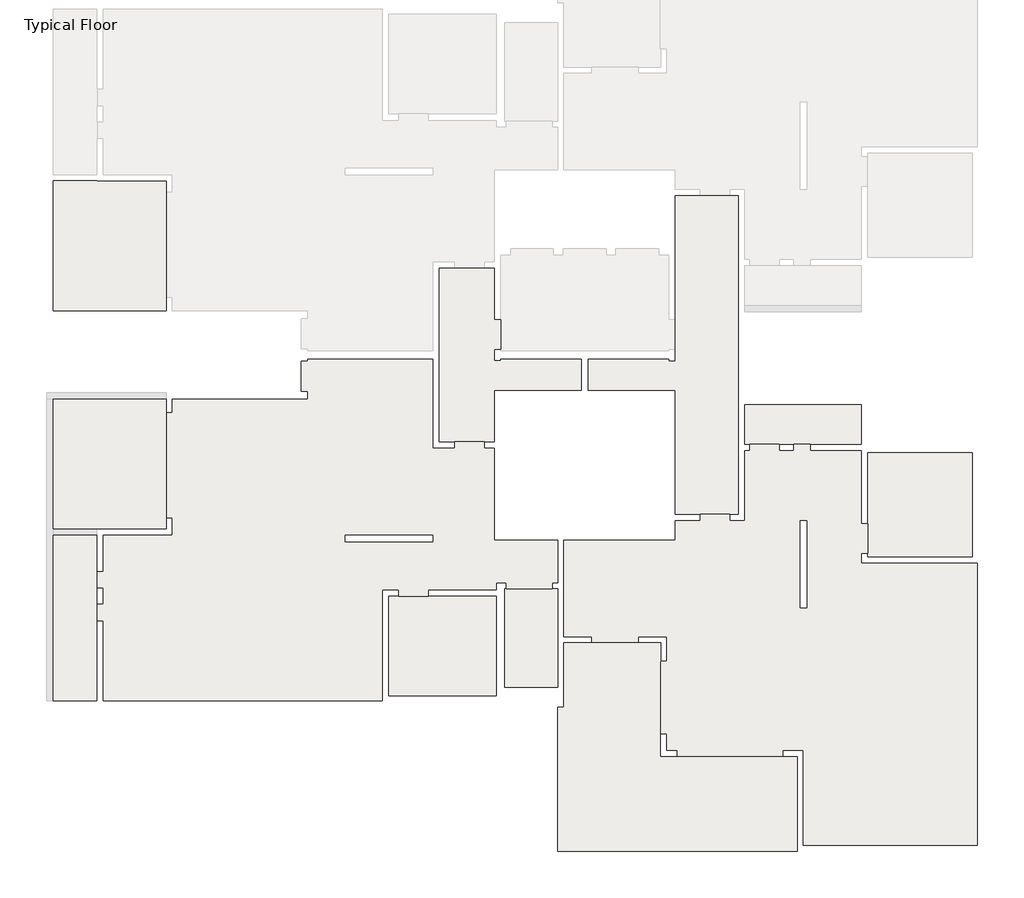
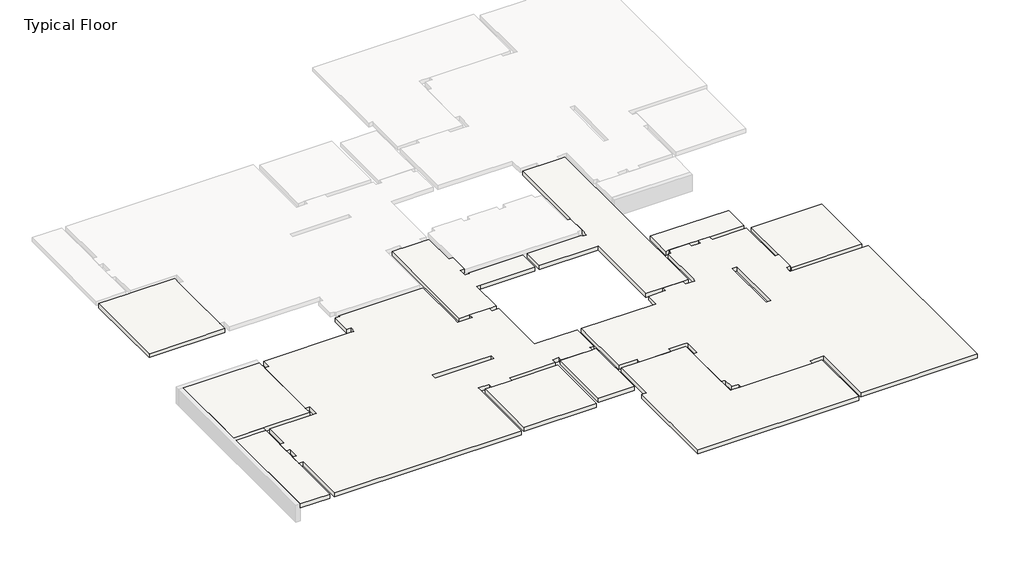
# One storey, part 1 of 2: 12 slabs.
"""IFC4 building model written with IfcOpenShell, lengths in millimetres."""

import ifcopenshell
import ifcopenshell.guid

model = None  # the IFC model being written
_history = None  # IfcOwnerHistory: only IFC2X3 demands one
_inside = {}  # id of a spatial element -> (the spatial element, [elements in it])
_under = {}  # id of a project, library or spatial element -> (it, [spatial elements below it])
_declared = {}  # id of a project -> (the project, [libraries it declares])
_typed = {}  # id of a type object -> (the type object, [elements of that type])
_made_of = {}  # id of a material, layer set ... -> (it, [elements and type objects made of it])


def new_model(schema):
    """Start an empty IFC model of exactly this schema.

    Asked for "IFC4X3", IfcOpenShell would pick the latest addendum, in which some entities
    have other attributes; the version numbers below select the first issue.
    IFC2X3 requires an IfcOwnerHistory on every rooted entity: one is made here for all.
    """
    global model, _history
    if schema == "IFC4X3":
        model = ifcopenshell.file(schema_version=(4, 3, 0, 0))
    else:
        model = ifcopenshell.file(schema=schema)
    _inside.clear()
    _under.clear()
    _declared.clear()
    _typed.clear()
    _made_of.clear()
    _history = None
    if model.schema == "IFC2X3":
        org = make("IfcOrganization", Name="unknown")
        user = make(
            "IfcPersonAndOrganization",
            ThePerson=make("IfcPerson", FamilyName="unknown"),
            TheOrganization=org,
        )
        app = make(
            "IfcApplication",
            ApplicationDeveloper=org,
            Version="unknown",
            ApplicationFullName="unknown",
            ApplicationIdentifier="unknown",
        )
        _history = make(
            "IfcOwnerHistory",
            OwningUser=user,
            OwningApplication=app,
            ChangeAction="ADDED",
            CreationDate=0,
        )
    return model


def make(cls, **values):
    """One entity of the class cls with the attributes given. An attribute that is None is left unset."""
    return model.create_entity(
        cls, **{name: value for name, value in values.items() if value is not None}
    )


def rooted(cls, **values):
    """An entity with a GlobalId (a new one), such as an element, a storey or a relation."""
    return make(cls, GlobalId=ifcopenshell.guid.new(), OwnerHistory=_history, **values)


def si_unit(unit_type, name, prefix=None):
    """IfcSIUnit, for example si_unit("LENGTHUNIT", "METRE", prefix="MILLI")."""
    return make("IfcSIUnit", UnitType=unit_type, Prefix=prefix, Name=name)


def assignment(units):
    """IfcUnitAssignment: the units of a project."""
    return None if units is None else make("IfcUnitAssignment", Units=units)


def point(xyz):
    """IfcCartesianPoint."""
    return None if xyz is None else make("IfcCartesianPoint", Coordinates=xyz)


def direction(xyz):
    """IfcDirection."""
    return None if xyz is None else make("IfcDirection", DirectionRatios=xyz)


def frame(location, z_axis=None, x_axis=None):
    """IfcAxis2Placement3D, a coordinate frame: its origin and axes. An axis left out is left unset."""
    return make(
        "IfcAxis2Placement3D",
        Location=point(location),
        Axis=direction(z_axis),
        RefDirection=direction(x_axis),
    )


def origin():
    """The frame at (0, 0, 0) with its axes left unset."""
    return frame((0.0, 0.0, 0.0))


def place(relative_to, where):
    """IfcLocalPlacement: puts the frame where relative to a parent placement (None: the world)."""
    return make(
        "IfcLocalPlacement", PlacementRelTo=relative_to, RelativePlacement=where
    )


def context(
    kind, dimensions, precision=None, world=None, true_north=None, identifier=None
):
    """IfcGeometricRepresentationContext, for example the 3D "Model" context."""
    return make(
        "IfcGeometricRepresentationContext",
        ContextIdentifier=identifier,
        ContextType=kind,
        CoordinateSpaceDimension=dimensions,
        Precision=precision,
        WorldCoordinateSystem=world,
        TrueNorth=true_north,
    )


def project(units=None, contexts=None):
    """IfcProject with its units and contexts."""
    return rooted(
        "IfcProject",
        Name="project",
        RepresentationContexts=contexts,
        UnitsInContext=assignment(units),
    )


def spatial(cls, under=None, at=None, **own):
    """A site, building, storey or space (cls), placed at a placement, below another one or the project."""
    s = rooted(cls, ObjectPlacement=at, **own)
    if under is not None:
        _under.setdefault(under.id(), (under, []))[1].append(s)
    return s


def faces_of(points, faces, orient=None, outer=None):
    """IfcFace entities. A face is a list of loops; a loop is a list of indices into points, from 0.

    orient and outer hold one flag for each loop. By default every Orientation is true, the
    first loop of a face is its IfcFaceOuterBound and the others are IfcFaceBound.
    """
    made = []
    for i, loops in enumerate(faces):
        bounds = []
        for j, loop in enumerate(loops):
            is_outer = j == 0 if outer is None else outer[i][j]
            bounds.append(
                make(
                    "IfcFaceOuterBound" if is_outer else "IfcFaceBound",
                    Bound=make("IfcPolyLoop", Polygon=[points[k] for k in loop]),
                    Orientation=True if orient is None else orient[i][j],
                )
            )
        made.append(make("IfcFace", Bounds=bounds))
    return made


def faceted_brep(points, faces, orient=None, outer=None, voids=None):
    """IfcFacetedBrep: a solid bounded by flat faces; with voids (closed shells), ...WithVoids."""
    shared = [point(p) for p in points]
    hull = make("IfcClosedShell", CfsFaces=faces_of(shared, faces, orient, outer))
    if voids is None:
        return make("IfcFacetedBrep", Outer=hull)
    return make(
        "IfcFacetedBrepWithVoids",
        Outer=hull,
        Voids=[
            make(cls, CfsFaces=faces_of(shared, fs, o, b)) for cls, fs, o, b in voids
        ],
    )


def shape(context_of_items, identifier, shape_type, items):
    """IfcShapeRepresentation: the items that make up one representation, for example the "Body"."""
    return make(
        "IfcShapeRepresentation",
        ContextOfItems=context_of_items,
        RepresentationIdentifier=identifier,
        RepresentationType=shape_type,
        Items=items,
    )


def made_of(thing, what):
    """Note that an element or type object is made of a material, layer set ...; save() writes the relation."""
    if what is not None:
        _made_of.setdefault(what.id(), (what, []))[1].append(thing)
    return thing


def element(
    cls,
    number,
    at=None,
    inside=None,
    cuts=None,
    type_object=None,
    material=None,
    context=None,
    identifier="Body",
    shape_type=None,
    held_by="IfcProductDefinitionShape",
    body=None,
    shapes=None,
    **own,
):
    """One element of the class cls, such as IfcWall. Its Tag is "e" and its number.

    at: its placement. inside: the storey or other place that contains it. cuts: it is an
    opening in that element (IfcRelVoidsElement). A single representation is given by context,
    identifier, shape_type and body (its items); several are given by shapes. held_by: the class
    of the entity that holds the representations. save() writes the other relations.
    """
    e = rooted(cls, Tag="e%d" % number, ObjectPlacement=at, **own)
    if body is not None:
        shapes = [shape(context, identifier, shape_type, body)]
    if shapes is not None:
        e.Representation = make(held_by, Representations=shapes)
    if inside is not None:
        _inside.setdefault(inside.id(), (inside, []))[1].append(e)
    if cuts is not None:
        rooted(
            "IfcRelVoidsElement", RelatingBuildingElement=cuts, RelatedOpeningElement=e
        )
    if type_object is not None:
        _typed.setdefault(type_object.id(), (type_object, []))[1].append(e)
    return made_of(e, material)


def aggregate(whole, parts):
    """IfcRelAggregates: a whole, such as a stair, and the parts it consists of."""
    return rooted("IfcRelAggregates", RelatingObject=whole, RelatedObjects=parts)


def save(model, path):
    """Write the relations noted so far, then the file.

    IfcRelAggregates (storeys below a building ...), IfcRelContainedInSpatialStructure (elements
    in a storey), IfcRelDefinesByType, IfcRelAssociatesMaterial and IfcRelDeclares: one each for
    every whole, place, type object, material and project.
    """
    for whole, parts in _under.values():
        aggregate(whole, parts)
    for where, things in _inside.values():
        rooted(
            "IfcRelContainedInSpatialStructure",
            RelatedElements=things,
            RelatingStructure=where,
        )
    for kind, things in _typed.values():
        rooted("IfcRelDefinesByType", RelatedObjects=things, RelatingType=kind)
    for what, things in _made_of.values():
        rooted("IfcRelAssociatesMaterial", RelatedObjects=things, RelatingMaterial=what)
    for by, libraries in _declared.values():
        rooted("IfcRelDeclares", RelatingContext=by, RelatedDefinitions=libraries)
    model.write(path)


model = new_model("IFC4")

# Units and contexts
model_context = context("Model", 3, world=origin())
ifc_project = project(units=[si_unit("LENGTHUNIT", "METRE", prefix="MILLI")], contexts=[model_context])

# Site, building, storey
site = spatial("IfcSite", under=ifc_project)
building = spatial("IfcBuilding", under=site)
storey = spatial("IfcBuildingStorey", under=building, Name="Typical Floor", Elevation=3000.0)

# Slabs
placement = place(None, origin())
element("IfcSlab", 1, ObjectType="19", at=placement, inside=storey, context=model_context, shape_type="Brep", body=[
    faceted_brep([(7776.7577342, 16126.4707233, 2810.0), (4344.3623691, 16126.4707233, 2810.0), (4344.3623691, 20058.0459905, 2810.0), (4344.3623691, 20073.0459905, 2810.0), (5676.0285364, 20073.0459905, 2810.0), (5676.0285364, 20058.0459905, 2810.0), (7776.7577342, 20058.0459905, 2810.0), (7776.7577342, 19727.6893828, 2810.0), (7776.7577342, 16527.889163, 2810.0), (4344.3623691, 16126.4707233, 3000.0), (7776.7577342, 16126.4707233, 3000.0), (7776.7577342, 16527.889163, 3000.0), (7776.7577342, 19727.6893828, 3000.0), (7776.7577342, 20058.0459905, 3000.0), (5866.0285364, 20058.0459905, 3000.0), (5676.0285364, 20058.0459905, 3000.0), (5676.0285364, 20073.0459905, 3000.0), (4344.3623691, 20073.0459905, 3000.0)], [[[0, 1, 2, 3, 4, 5, 6, 7, 8]], [[9, 10, 11, 12, 13, 14, 15, 16, 17]], [[3, 17, 16, 4]], [[10, 0, 8, 7, 6, 13, 12, 11]], [[1, 0, 10, 9]], [[3, 2, 1, 9, 17]], [[5, 15, 14, 13, 6]], [[15, 5, 4, 16]]]),
])
element("IfcSlab", 2, ObjectType="19", at=placement, inside=storey, context=model_context, shape_type="Brep", body=[
    faceted_brep([(4344.3623691, 9503.461034, 2810.0), (4344.3623691, 13435.0363012, 2810.0), (7776.7577342, 13435.0363012, 2810.0), (7776.7577342, 13033.6178615, 2810.0), (7776.7577342, 9833.8176417, 2810.0), (7776.7577342, 9503.461034, 2810.0), (4344.3623691, 9503.461034, 3000.0), (5676.0285364, 9503.461034, 3000.0), (5866.0285364, 9503.461034, 3000.0), (7776.7577342, 9503.461034, 3000.0), (7776.7577342, 9833.8176417, 3000.0), (7776.7577342, 13033.6178615, 3000.0), (7776.7577342, 13435.0363012, 3000.0), (4344.3623691, 13435.0363012, 3000.0)], [[[0, 1, 2, 3, 4, 5]], [[6, 7, 8, 9, 10, 11, 12, 13]], [[0, 5, 9, 8, 7, 6]], [[5, 4, 3, 2, 12, 11, 10, 9]], [[2, 1, 13, 12]], [[1, 0, 6, 13]]]),
])
element("IfcSlab", 3, ObjectType="19", at=placement, inside=storey, context=model_context, shape_type="Brep", body=[
    faceted_brep([(5676.0285364, 4280.8870961, 2810.0), (4344.3623691, 4280.8870961, 2810.0), (4344.3623691, 9303.461034, 2810.0), (4344.3623691, 9308.461034, 2810.0), (5676.0285364, 9308.461034, 2810.0), (5676.0285364, 9303.461034, 2810.0), (5676.0285364, 8207.3295478, 2810.0), (5676.0285364, 7708.0987786, 2810.0), (5676.0285364, 7208.8680094, 2810.0), (5676.0285364, 6709.6372401, 2810.0), (5676.0285364, 4280.8870961, 3000.0), (5676.0285364, 6709.6372401, 3000.0), (5676.0285364, 7208.8680094, 3000.0), (5676.0285364, 7708.0987786, 3000.0), (5676.0285364, 8207.3295478, 3000.0), (5676.0285364, 9308.461034, 3000.0), (4344.3623691, 9308.461034, 3000.0), (4344.3623691, 4280.8870961, 3000.0)], [[[0, 1, 2, 3, 4, 5, 6, 7, 8, 9]], [[10, 11, 12, 13, 14, 15, 16, 17]], [[0, 9, 8, 7, 6, 5, 4, 15, 14, 13, 12, 11, 10]], [[4, 3, 16, 15]], [[3, 2, 1, 17, 16]], [[1, 0, 10, 17]]]),
])
element("IfcSlab", 4, ObjectType="19", at=placement, inside=storey, context=model_context, shape_type="Brep", body=[
    faceted_brep([(5866.0285364, 4280.8870961, 2810.0), (5866.0285364, 6709.6372401, 2810.0), (5676.0285364, 6709.6372401, 2810.0), (5676.0285364, 7208.8680094, 2810.0), (5866.0285364, 7208.8680094, 2810.0), (5866.0285364, 7708.0987786, 2810.0), (5676.0285364, 7708.0987786, 2810.0), (5676.0285364, 8207.3295478, 2810.0), (5866.0285364, 8207.3295478, 2810.0), (5866.0285364, 9313.461034, 2810.0), (7776.7577342, 9313.461034, 2810.0), (7966.7577342, 9313.461034, 2810.0), (7966.7577342, 9833.8176417, 2810.0), (7776.7577342, 9833.8176417, 2810.0), (7776.7577342, 13033.6178615, 2810.0), (7966.7577342, 13033.6178615, 2810.0), (7966.7577342, 13435.0363012, 2810.0), (11878.6856136, 13435.0363012, 2810.0), (12068.6856136, 13435.0363012, 2810.0), (12068.6856136, 13683.7427241, 2810.0), (11878.6856136, 13683.7427241, 2810.0), (11878.6856136, 14585.8703837, 2810.0), (12068.6856136, 14585.8703837, 2810.0), (12068.6856136, 14655.7535122, 2810.0), (15871.0829765, 14655.7535122, 2810.0), (15871.0829765, 12153.6058746, 2810.0), (15871.0829765, 11953.6058746, 2810.0), (16530.6174885, 11953.6058746, 2810.0), (16530.6174885, 12153.6058746, 2810.0), (17430.6274775, 12153.6058746, 2810.0), (17430.6274775, 11953.6058746, 2810.0), (17731.3366974, 11953.6058746, 2810.0), (17731.3366974, 9151.9277206, 2810.0), (17931.3366974, 9151.9277206, 2810.0), (19662.6522503, 9151.9277206, 2810.0), (19662.6522503, 7872.8547009, 2810.0), (19501.7092875, 7872.8547009, 2810.0), (19501.7092875, 7682.8547009, 2810.0), (18101.9290458, 7682.8547009, 2810.0), (18101.9290458, 7872.8547009, 2810.0), (18051.1049523, 7872.8547009, 2810.0), (17801.1049523, 7872.8547009, 2810.0), (17801.1049523, 7661.0876447, 2810.0), (15730.1380159, 7661.0876447, 2810.0), (15730.1380159, 7461.0876447, 2810.0), (14830.1280269, 7461.0876447, 2810.0), (14830.1280269, 7661.0876447, 2810.0), (14329.4188071, 7661.0876447, 2810.0), (14329.4188071, 7461.0876447, 2810.0), (14329.4188071, 4280.8870961, 2810.0), (13218.5807289, 9112.8706834, 2810.0), (15869.904273, 9112.8706834, 2810.0), (15869.904273, 9312.8706834, 2810.0), (13218.5807289, 9312.8706834, 2810.0), (5866.0285364, 6709.6372401, 3000.0), (5866.0285364, 4280.8870961, 3000.0), (14329.4188071, 4280.8870961, 3000.0), (14329.4188071, 7461.0876447, 3000.0), (14329.4188071, 7661.0876447, 3000.0), (14830.1280269, 7661.0876447, 3000.0), (14830.1280269, 7461.0876447, 3000.0), (15730.1380159, 7461.0876447, 3000.0), (15730.1380159, 7661.0876447, 3000.0), (17801.1049523, 7661.0876447, 3000.0), (17801.1049523, 7872.8547009, 3000.0), (18051.1049523, 7872.8547009, 3000.0), (18101.9290458, 7872.8547009, 3000.0), (18101.9290458, 7682.8547009, 3000.0), (19501.7092875, 7682.8547009, 3000.0), (19501.7092875, 7872.8547009, 3000.0), (19662.6522503, 7872.8547009, 3000.0), (19662.6522503, 9151.9277206, 3000.0), (17931.3366974, 9151.9277206, 3000.0), (17731.3366974, 9151.9277206, 3000.0), (17731.3366974, 11953.6058746, 3000.0), (17430.6274775, 11953.6058746, 3000.0), (17430.6274775, 12153.6058746, 3000.0), (16530.6174885, 12153.6058746, 3000.0), (16530.6174885, 11953.6058746, 3000.0), (15871.0829765, 11953.6058746, 3000.0), (15871.0829765, 12153.6058746, 3000.0), (15871.0829765, 14655.7535122, 3000.0), (12068.6856136, 14655.7535122, 3000.0), (12068.6856136, 14585.8703837, 3000.0), (11878.6856136, 14585.8703837, 3000.0), (11878.6856136, 13683.7427241, 3000.0), (12068.6856136, 13683.7427241, 3000.0), (12068.6856136, 13435.0363012, 3000.0), (11878.6856136, 13435.0363012, 3000.0), (7966.7577342, 13435.0363012, 3000.0), (7966.7577342, 13033.6178615, 3000.0), (7776.7577342, 13033.6178615, 3000.0), (7776.7577342, 9833.8176417, 3000.0), (7966.7577342, 9833.8176417, 3000.0), (7966.7577342, 9313.461034, 3000.0), (7776.7577342, 9313.461034, 3000.0), (5866.0285364, 9313.461034, 3000.0), (5866.0285364, 8207.3295478, 3000.0), (5676.0285364, 8207.3295478, 3000.0), (5676.0285364, 7708.0987786, 3000.0), (5866.0285364, 7708.0987786, 3000.0), (5866.0285364, 7208.8680094, 3000.0), (5676.0285364, 7208.8680094, 3000.0), (5676.0285364, 6709.6372401, 3000.0), (15869.904273, 9112.8706834, 3000.0), (13218.5807289, 9112.8706834, 3000.0), (13218.5807289, 9312.8706834, 3000.0), (15869.904273, 9312.8706834, 3000.0)], [[[0, 1, 2, 3, 4, 5, 6, 7, 8, 9, 10, 11, 12, 13, 14, 15, 16, 17, 18, 19, 20, 21, 22, 23, 24, 25, 26, 27, 28, 29, 30, 31, 32, 33, 34, 35, 36, 37, 38, 39, 40, 41, 42, 43, 44, 45, 46, 47, 48, 49], [50, 51, 52, 53]], [[54, 55, 56, 57, 58, 59, 60, 61, 62, 63, 64, 65, 66, 67, 68, 69, 70, 71, 72, 73, 74, 75, 76, 77, 78, 79, 80, 81, 82, 83, 84, 85, 86, 87, 88, 89, 90, 91, 92, 93, 94, 95, 96, 97, 98, 99, 100, 101, 102, 103], [104, 105, 106, 107]], [[1, 0, 55, 54]], [[0, 49, 56, 55]], [[47, 58, 57, 56, 49, 48]], [[47, 46, 59, 58]], [[46, 45, 60, 59]], [[45, 44, 61, 60]], [[44, 43, 62, 61]], [[43, 42, 63, 62]], [[42, 41, 64, 63]], [[39, 66, 65, 64, 41, 40]], [[39, 38, 67, 66]], [[38, 37, 68, 67]], [[37, 36, 69, 68]], [[36, 35, 70, 69]], [[35, 34, 71, 70]], [[32, 73, 72, 71, 34, 33]], [[32, 31, 74, 73]], [[31, 30, 75, 74]], [[30, 29, 76, 75]], [[29, 28, 77, 76]], [[28, 27, 78, 77]], [[27, 26, 79, 78]], [[24, 81, 80, 79, 26, 25]], [[24, 23, 82, 81]], [[23, 22, 83, 82]], [[22, 21, 84, 83]], [[21, 20, 85, 84]], [[20, 19, 86, 85]], [[19, 18, 87, 86]], [[16, 89, 88, 87, 18, 17]], [[16, 15, 90, 89]], [[15, 14, 91, 90]], [[14, 13, 92, 91]], [[13, 12, 93, 92]], [[12, 11, 94, 93]], [[9, 96, 95, 94, 11, 10]], [[9, 8, 97, 96]], [[8, 7, 98, 97]], [[7, 6, 99, 98]], [[6, 5, 100, 99]], [[5, 4, 101, 100]], [[4, 3, 102, 101]], [[3, 2, 103, 102]], [[2, 1, 54, 103]], [[51, 50, 105, 104]], [[50, 53, 106, 105]], [[53, 52, 107, 106]], [[52, 51, 104, 107]]]),
])
element("IfcSlab", 5, ObjectType="19", at=placement, inside=storey, context=model_context, shape_type="Brep", body=[
    faceted_brep([(19852.6522503, 9151.9277206, 2810.0), (23233.0448184, 9151.9277206, 2810.0), (23233.0448184, 9351.9277206, 2810.0), (23233.0448184, 9752.4071932, 2810.0), (23984.8178681, 9752.4071932, 2810.0), (23984.8178681, 9952.4071932, 2810.0), (24884.8278571, 9952.4071932, 2810.0), (24884.8278571, 9752.4071932, 2810.0), (25344.8278571, 9752.4071932, 2810.0), (25344.8278571, 9952.4071932, 2810.0), (25344.8278571, 11873.1343933, 2810.0), (25494.7169791, 11873.1343933, 2810.0), (25494.7169791, 12073.1343933, 2810.0), (26394.7269681, 12073.1343933, 2810.0), (26394.7269681, 11873.1343933, 2810.0), (26824.6140922, 11873.1343933, 2810.0), (26824.6140922, 12073.1343933, 2810.0), (27326.5020155, 12073.1343933, 2810.0), (27326.5020155, 11873.1343933, 2810.0), (28876.6368672, 11873.1343933, 2810.0), (28876.6368672, 9662.2863261, 2810.0), (29076.6368672, 9662.2863261, 2810.0), (29076.6368672, 8762.2763371, 2810.0), (28876.6368672, 8762.2763371, 2810.0), (28876.6368672, 8461.5671173, 2810.0), (29076.6368672, 8461.5671173, 2810.0), (32407.3840453, 8461.5671173, 2810.0), (32407.3840453, -100.765317, 2810.0), (27124.7329615, -100.765317, 2810.0), (27124.7329615, 2589.8569984, 2810.0), (27124.7329615, 2779.8569984, 2810.0), (26490.0221434, 2779.8569984, 2810.0), (26490.0221434, 2589.8569984, 2810.0), (23288.1042531, 2589.8569984, 2810.0), (23288.1042531, 2779.8569984, 2810.0), (22974.0986592, 2779.8569984, 2810.0), (22974.0986592, 3279.6272511, 2810.0), (22784.0986592, 3279.6272511, 2810.0), (22784.0986592, 5479.8869654, 2810.0), (22784.6890098, 5479.8869654, 2810.0), (22974.6890098, 5479.8869654, 2810.0), (22974.6890098, 6231.6600151, 2810.0), (22784.6890098, 6231.6600151, 2810.0), (22104.3264087, 6231.6600151, 2810.0), (22104.3264087, 6041.6600151, 2810.0), (20702.4284964, 6041.6600151, 2810.0), (20702.4284964, 6231.6600151, 2810.0), (19852.6522503, 6231.6600151, 2810.0), (27025.7927957, 9753.3461603, 2810.0), (27025.7927957, 7102.0226162, 2810.0), (27225.7927957, 7102.0226162, 2810.0), (27225.7927957, 9753.3461603, 2810.0), (23233.0448184, 9151.9277206, 3000.0), (19852.6522503, 9151.9277206, 3000.0), (19852.6522503, 6231.6600151, 3000.0), (20702.4284964, 6231.6600151, 3000.0), (20702.4284964, 6041.6600151, 3000.0), (22104.3264087, 6041.6600151, 3000.0), (22104.3264087, 6231.6600151, 3000.0), (22784.6890098, 6231.6600151, 3000.0), (22974.6890098, 6231.6600151, 3000.0), (22974.6890098, 5479.8869654, 3000.0), (22784.6890098, 5479.8869654, 3000.0), (22784.0986592, 5479.8869654, 3000.0), (22784.0986592, 3279.6272511, 3000.0), (22974.0986592, 3279.6272511, 3000.0), (22974.0986592, 2779.8569984, 3000.0), (23288.1042531, 2779.8569984, 3000.0), (23288.1042531, 2589.8569984, 3000.0), (26490.0221434, 2589.8569984, 3000.0), (26490.0221434, 2779.8569984, 3000.0), (27124.7329615, 2779.8569984, 3000.0), (27124.7329615, 2589.8569984, 3000.0), (27124.7329615, -100.765317, 3000.0), (32407.3840453, -100.765317, 3000.0), (32407.3840453, 8461.5671173, 3000.0), (29076.6368672, 8461.5671173, 3000.0), (28876.6368672, 8461.5671173, 3000.0), (28876.6368672, 8762.2763371, 3000.0), (29076.6368672, 8762.2763371, 3000.0), (29076.6368672, 9662.2863261, 3000.0), (28876.6368672, 9662.2863261, 3000.0), (28876.6368672, 11873.1343933, 3000.0), (27326.5020155, 11873.1343933, 3000.0), (27326.5020155, 12073.1343933, 3000.0), (26824.6140922, 12073.1343933, 3000.0), (26824.6140922, 11873.1343933, 3000.0), (26394.7269681, 11873.1343933, 3000.0), (26394.7269681, 12073.1343933, 3000.0), (25494.7169791, 12073.1343933, 3000.0), (25494.7169791, 11873.1343933, 3000.0), (25344.8278571, 11873.1343933, 3000.0), (25344.8278571, 9952.4071932, 3000.0), (25344.8278571, 9752.4071932, 3000.0), (24884.8278571, 9752.4071932, 3000.0), (24884.8278571, 9952.4071932, 3000.0), (23984.8178681, 9952.4071932, 3000.0), (23984.8178681, 9752.4071932, 3000.0), (23233.0448184, 9752.4071932, 3000.0), (23233.0448184, 9351.9277206, 3000.0), (27025.7927957, 7102.0226162, 3000.0), (27025.7927957, 9753.3461603, 3000.0), (27225.7927957, 9753.3461603, 3000.0), (27225.7927957, 7102.0226162, 3000.0)], [[[0, 1, 2, 3, 4, 5, 6, 7, 8, 9, 10, 11, 12, 13, 14, 15, 16, 17, 18, 19, 20, 21, 22, 23, 24, 25, 26, 27, 28, 29, 30, 31, 32, 33, 34, 35, 36, 37, 38, 39, 40, 41, 42, 43, 44, 45, 46, 47], [48, 49, 50, 51]], [[52, 53, 54, 55, 56, 57, 58, 59, 60, 61, 62, 63, 64, 65, 66, 67, 68, 69, 70, 71, 72, 73, 74, 75, 76, 77, 78, 79, 80, 81, 82, 83, 84, 85, 86, 87, 88, 89, 90, 91, 92, 93, 94, 95, 96, 97, 98, 99], [100, 101, 102, 103]], [[1, 0, 53, 52]], [[0, 47, 54, 53]], [[47, 46, 55, 54]], [[46, 45, 56, 55]], [[45, 44, 57, 56]], [[44, 43, 58, 57]], [[41, 60, 59, 58, 43, 42]], [[41, 40, 61, 60]], [[38, 63, 62, 61, 40, 39]], [[38, 37, 64, 63]], [[37, 36, 65, 64]], [[36, 35, 66, 65]], [[35, 34, 67, 66]], [[34, 33, 68, 67]], [[33, 32, 69, 68]], [[32, 31, 70, 69]], [[31, 30, 71, 70]], [[28, 73, 72, 71, 30, 29]], [[28, 27, 74, 73]], [[27, 26, 75, 74]], [[24, 77, 76, 75, 26, 25]], [[24, 23, 78, 77]], [[23, 22, 79, 78]], [[22, 21, 80, 79]], [[21, 20, 81, 80]], [[20, 19, 82, 81]], [[19, 18, 83, 82]], [[18, 17, 84, 83]], [[17, 16, 85, 84]], [[16, 15, 86, 85]], [[15, 14, 87, 86]], [[14, 13, 88, 87]], [[13, 12, 89, 88]], [[12, 11, 90, 89]], [[11, 10, 91, 90]], [[8, 93, 92, 91, 10, 9]], [[8, 7, 94, 93]], [[7, 6, 95, 94]], [[6, 5, 96, 95]], [[5, 4, 97, 96]], [[4, 3, 98, 97]], [[98, 3, 2, 1, 52, 99]], [[48, 101, 100, 49]], [[50, 103, 102, 51]], [[49, 100, 103, 50]], [[101, 48, 51, 102]]]),
])
element("IfcSlab", 6, ObjectType="19", at=placement, inside=storey, context=model_context, shape_type="Brep", body=[
    faceted_brep([(32247.3840453, 8661.5671173, 2810.0), (29076.6368672, 8661.5671173, 2810.0), (29076.6368672, 8762.2763371, 2810.0), (29076.6368672, 9662.2863261, 2810.0), (29076.6368672, 11813.7247439, 2810.0), (32247.3840453, 11813.7247439, 2810.0), (29076.6368672, 8661.5671173, 3000.0), (32247.3840453, 8661.5671173, 3000.0), (32247.3840453, 11813.7247439, 3000.0), (29076.6368672, 11813.7247439, 3000.0), (29076.6368672, 9662.2863261, 3000.0), (29076.6368672, 8762.2763371, 3000.0)], [[[0, 1, 2, 3, 4, 5]], [[6, 7, 8, 9, 10, 11]], [[1, 0, 7, 6]], [[0, 5, 8, 7]], [[5, 4, 9, 8]], [[9, 4, 3, 2, 1, 6, 11, 10]]]),
])
element("IfcSlab", 7, ObjectType="19", at=placement, inside=storey, context=model_context, shape_type="Brep", body=[
    faceted_brep([(26934.7329615, -290.765317, 2810.0), (19662.6522503, -290.765317, 2810.0), (19662.6522503, 4090.6950765, 2810.0), (19852.6522503, 4090.6950765, 2810.0), (19852.6522503, 6041.6600151, 2810.0), (20702.4284964, 6041.6600151, 2810.0), (22104.3264087, 6041.6600151, 2810.0), (22784.6890098, 6041.6600151, 2810.0), (22784.6890098, 5479.8869654, 2810.0), (22784.0986592, 5479.8869654, 2810.0), (22784.0986592, 3279.6272511, 2810.0), (22784.0986592, 2589.8569984, 2810.0), (23288.1042531, 2589.8569984, 2810.0), (26490.0221434, 2589.8569984, 2810.0), (26934.7329615, 2589.8569984, 2810.0), (19662.6522503, -290.765317, 3000.0), (26934.7329615, -290.765317, 3000.0), (26934.7329615, -100.765317, 3000.0), (26934.7329615, 2589.8569984, 3000.0), (26490.0221434, 2589.8569984, 3000.0), (23288.1042531, 2589.8569984, 3000.0), (22974.0986592, 2589.8569984, 3000.0), (22784.0986592, 2589.8569984, 3000.0), (22784.0986592, 3279.6272511, 3000.0), (22784.0986592, 5479.8869654, 3000.0), (22784.6890098, 5479.8869654, 3000.0), (22784.6890098, 6041.6600151, 3000.0), (22104.3264087, 6041.6600151, 3000.0), (20702.4284964, 6041.6600151, 3000.0), (19852.6522503, 6041.6600151, 3000.0), (19852.6522503, 4090.6950765, 3000.0), (19662.6522503, 4090.6950765, 3000.0)], [[[0, 1, 2, 3, 4, 5, 6, 7, 8, 9, 10, 11, 12, 13, 14]], [[15, 16, 17, 18, 19, 20, 21, 22, 23, 24, 25, 26, 27, 28, 29, 30, 31]], [[1, 0, 16, 15]], [[0, 14, 18, 17, 16]], [[18, 14, 13, 12, 11, 22, 21, 20, 19]], [[3, 30, 29, 4]], [[3, 2, 31, 30]], [[2, 1, 15, 31]], [[22, 11, 10, 9, 24, 23]], [[8, 7, 26, 25]], [[26, 7, 6, 5, 4, 29, 28, 27]], [[24, 9, 8, 25]]]),
])
element("IfcSlab", 8, ObjectType="19", at=placement, inside=storey, context=model_context, shape_type="Brep", body=[
    faceted_brep([(14529.4188071, 4440.7910863, 2810.0), (14529.4188071, 7461.0876447, 2810.0), (14830.1280269, 7461.0876447, 2810.0), (15730.1380159, 7461.0876447, 2810.0), (17801.1049523, 7461.0876447, 2810.0), (17801.1049523, 4440.7910863, 2810.0), (14529.4188071, 7461.0876447, 3000.0), (14529.4188071, 4440.7910863, 3000.0), (17801.1049523, 4440.7910863, 3000.0), (17801.1049523, 7461.0876447, 3000.0), (15730.1380159, 7461.0876447, 3000.0), (14830.1280269, 7461.0876447, 3000.0)], [[[0, 1, 2, 3, 4, 5]], [[6, 7, 8, 9, 10, 11]], [[1, 6, 11, 10, 9, 4, 3, 2]], [[1, 0, 7, 6]], [[0, 5, 8, 7]], [[5, 4, 9, 8]]]),
])
element("IfcSlab", 9, ObjectType="19", at=placement, inside=storey, context=model_context, shape_type="Brep", body=[
    faceted_brep([(17731.3366974, 17407.9011498, 2810.0), (17731.3366974, 15852.9011498, 2810.0), (17931.3366974, 15852.9011498, 2810.0), (17931.3366974, 14956.5776057, 2810.0), (17731.3366974, 14956.5776057, 2810.0), (17731.3366974, 14607.1619629, 2810.0), (17931.3366974, 14607.1619629, 2810.0), (17931.3366974, 14655.8683859, 2810.0), (20384.2581025, 14655.8683859, 2810.0), (20384.2581025, 13708.6058746, 2810.0), (17931.3366974, 13708.6058746, 2810.0), (17731.3366974, 13708.6058746, 2810.0), (17731.3366974, 12153.6058746, 2810.0), (17430.6274775, 12153.6058746, 2810.0), (16530.6174885, 12153.6058746, 2810.0), (16071.0829765, 12153.6058746, 2810.0), (16071.0829765, 17407.9011498, 2810.0), (16530.6174885, 17407.9011498, 2810.0), (17430.6274775, 17407.9011498, 2810.0), (17731.3366974, 15852.9011498, 3000.0), (17731.3366974, 17407.9011498, 3000.0), (17430.6274775, 17407.9011498, 3000.0), (16530.6174885, 17407.9011498, 3000.0), (16071.0829765, 17407.9011498, 3000.0), (16071.0829765, 12153.6058746, 3000.0), (16530.6174885, 12153.6058746, 3000.0), (17430.6274775, 12153.6058746, 3000.0), (17731.3366974, 12153.6058746, 3000.0), (17731.3366974, 13708.6058746, 3000.0), (17931.3366974, 13708.6058746, 3000.0), (20384.2581025, 13708.6058746, 3000.0), (20384.2581025, 14655.8683859, 3000.0), (17931.3366974, 14655.8683859, 3000.0), (17931.3366974, 14607.1619629, 3000.0), (17731.3366974, 14607.1619629, 3000.0), (17731.3366974, 14956.5776057, 3000.0), (17931.3366974, 14956.5776057, 3000.0), (17931.3366974, 15852.9011498, 3000.0)], [[[0, 1, 2, 3, 4, 5, 6, 7, 8, 9, 10, 11, 12, 13, 14, 15, 16, 17, 18]], [[19, 20, 21, 22, 23, 24, 25, 26, 27, 28, 29, 30, 31, 32, 33, 34, 35, 36, 37]], [[23, 16, 15, 24]], [[16, 23, 22, 21, 20, 0, 18, 17]], [[1, 0, 20, 19]], [[2, 1, 19, 37]], [[3, 2, 37, 36]], [[4, 3, 36, 35]], [[5, 4, 35, 34]], [[6, 5, 34, 33]], [[7, 6, 33, 32]], [[8, 7, 32, 31]], [[9, 8, 31, 30]], [[10, 9, 30, 29]], [[11, 10, 29, 28]], [[11, 28, 27, 12]], [[24, 15, 14, 13, 12, 27, 26, 25]]]),
])
element("IfcSlab", 10, ObjectType="19", at=placement, inside=storey, context=model_context, shape_type="Brep", body=[
    faceted_brep([(20584.2581025, 13704.9194297, 2810.0), (20584.2581025, 14655.8683859, 2810.0), (23033.0448184, 14655.8683859, 2810.0), (23033.0448184, 14596.5776057, 2810.0), (23233.0448184, 14596.5776057, 2810.0), (23233.0448184, 14956.5776057, 2810.0), (23233.0448184, 15856.5875947, 2810.0), (23233.0448184, 19609.0998313, 2810.0), (23984.8178681, 19609.0998313, 2810.0), (24884.8278571, 19609.0998313, 2810.0), (25144.8278571, 19609.0998313, 2810.0), (25144.8278571, 9952.4071932, 2810.0), (24884.8278571, 9952.4071932, 2810.0), (23984.8178681, 9952.4071932, 2810.0), (23233.0448184, 9952.4071932, 2810.0), (23233.0448184, 13704.9194297, 2810.0), (23033.0448184, 13704.9194297, 2810.0), (20584.2581025, 14655.8683859, 3000.0), (20584.2581025, 13704.9194297, 3000.0), (23033.0448184, 13704.9194297, 3000.0), (23233.0448184, 13704.9194297, 3000.0), (23233.0448184, 9952.4071932, 3000.0), (23984.8178681, 9952.4071932, 3000.0), (24884.8278571, 9952.4071932, 3000.0), (25144.8278571, 9952.4071932, 3000.0), (25144.8278571, 19609.0998313, 3000.0), (24884.8278571, 19609.0998313, 3000.0), (23984.8178681, 19609.0998313, 3000.0), (23233.0448184, 19609.0998313, 3000.0), (23233.0448184, 15856.5875947, 3000.0), (23233.0448184, 14956.5776057, 3000.0), (23233.0448184, 14596.5776057, 3000.0), (23033.0448184, 14596.5776057, 3000.0), (23033.0448184, 14655.8683859, 3000.0)], [[[0, 1, 2, 3, 4, 5, 6, 7, 8, 9, 10, 11, 12, 13, 14, 15, 16]], [[17, 18, 19, 20, 21, 22, 23, 24, 25, 26, 27, 28, 29, 30, 31, 32, 33]], [[28, 7, 6, 5, 4, 31, 30, 29]], [[7, 28, 27, 26, 25, 10, 9, 8]], [[10, 25, 24, 11]], [[20, 15, 14, 21]], [[15, 20, 19, 18, 0, 16]], [[1, 0, 18, 17]], [[2, 1, 17, 33]], [[3, 2, 33, 32]], [[4, 3, 32, 31]], [[21, 14, 13, 12, 11, 24, 23, 22]]]),
])
element("IfcSlab", 11, ObjectType="19", at=placement, inside=storey, context=model_context, shape_type="Brep", body=[
    faceted_brep([(19662.6522503, 7682.8547009, 2810.0), (19662.6522503, 4692.2283899, 2810.0), (18051.1049523, 4692.2283899, 2810.0), (18051.1049523, 7682.8547009, 2810.0), (18101.9290458, 7682.8547009, 2810.0), (19501.7092875, 7682.8547009, 2810.0), (19662.6522503, 4692.2283899, 3000.0), (19662.6522503, 7682.8547009, 3000.0), (19501.7092875, 7682.8547009, 3000.0), (18101.9290458, 7682.8547009, 3000.0), (18051.1049523, 7682.8547009, 3000.0), (18051.1049523, 7461.0876447, 3000.0), (18051.1049523, 4692.2283899, 3000.0)], [[[0, 1, 2, 3, 4, 5]], [[6, 7, 8, 9, 10, 11, 12]], [[1, 0, 7, 6]], [[1, 6, 12, 2]], [[7, 0, 5, 4, 3, 10, 9, 8]], [[2, 12, 11, 10, 3]]]),
])
element("IfcSlab", 12, ObjectType="19", at=placement, inside=storey, context=model_context, shape_type="Brep", body=[
    faceted_brep([(28875.6979001, 13264.5588264, 2810.0), (28875.6979001, 12073.1343933, 2810.0), (27326.5020155, 12073.1343933, 2810.0), (26824.6140922, 12073.1343933, 2810.0), (26394.7269681, 12073.1343933, 2810.0), (25494.7169791, 12073.1343933, 2810.0), (25344.8278571, 12073.1343933, 2810.0), (25344.8278571, 13264.5588264, 2810.0), (28875.6979001, 13264.5588264, 3000.0), (25344.8278571, 13264.5588264, 3000.0), (25344.8278571, 12073.1343933, 3000.0), (25494.7169791, 12073.1343933, 3000.0), (26394.7269681, 12073.1343933, 3000.0), (26824.6140922, 12073.1343933, 3000.0), (27326.5020155, 12073.1343933, 3000.0), (28875.6979001, 12073.1343933, 3000.0)], [[[0, 1, 2, 3, 4, 5, 6, 7]], [[8, 9, 10, 11, 12, 13, 14, 15]], [[1, 0, 8, 15]], [[6, 5, 4, 3, 2, 1, 15, 14, 13, 12, 11, 10]], [[7, 6, 10, 9]], [[0, 7, 9, 8]]]),
])

save(model, "model.ifc")

# Revit data of these elements
# Type "19"
#   Function = 0
#   Layers, outside or top first: 19 cm "Concrete" (function 1)
# Element 1 (IfcSlab, "19")
#   Mark = "S1"
#   SOFiSTiK_AMG_Comments = ""
#   built-in parameter 1001955 = 3.14159 (stored number, unit not read)
#   Height Offset From Level = 0 cm
#   built-in parameter 1001954 = 1
#   SOFiSTiK_AMG_Scheduled = yes
#   SOFiSTiK_AMG_Adjusted = yes
#   Phase Created = New Construction
#   Materials on its faces: "Concrete"
# Element 2 (IfcSlab, "19")
#   Mark = "S8"
#   SOFiSTiK_AMG_Comments = ""
#   built-in parameter 1001955 = 3.14159 (stored number, unit not read)
#   Height Offset From Level = 0 cm
#   built-in parameter 1001954 = 1
#   SOFiSTiK_AMG_Scheduled = yes
#   SOFiSTiK_AMG_Adjusted = yes
#   Phase Created = New Construction
#   Materials on its faces: "Concrete"
# Element 3 (IfcSlab, "19")
#   Mark = "S9"
#   SOFiSTiK_AMG_Comments = ""
#   Height Offset From Level = 0 cm
#   built-in parameter 1001954 = 1
#   SOFiSTiK_AMG_Scheduled = yes
#   SOFiSTiK_AMG_Adjusted = yes
#   Phase Created = New Construction
#   Materials on its faces: "Concrete"
# Element 4 (IfcSlab, "19")
#   Mark = "S10"
#   SOFiSTiK_AMG_Comments = ""
#   built-in parameter 1001955 = 1.5708 (stored number, unit not read)
#   Height Offset From Level = 0 cm
#   built-in parameter 1001954 = 1
#   SOFiSTiK_AMG_Scheduled = yes
#   SOFiSTiK_AMG_Adjusted = yes
#   Phase Created = New Construction
#   Materials on its faces: "Concrete"
# Element 5 (IfcSlab, "19")
#   Mark = "S11"
#   SOFiSTiK_AMG_Comments = ""
#   Height Offset From Level = 0 cm
#   built-in parameter 1001954 = 1
#   SOFiSTiK_AMG_Scheduled = yes
#   SOFiSTiK_AMG_Adjusted = yes
#   Phase Created = New Construction
#   Materials on its faces: "Concrete"
# Element 6 (IfcSlab, "19")
#   Mark = "S12"
#   SOFiSTiK_AMG_Comments = ""
#   built-in parameter 1001955 = 3.14159 (stored number, unit not read)
#   Height Offset From Level = 0 cm
#   built-in parameter 1001954 = 1
#   SOFiSTiK_AMG_Scheduled = yes
#   SOFiSTiK_AMG_Adjusted = yes
#   Phase Created = New Construction
#   Materials on its faces: "Concrete"
# Element 7 (IfcSlab, "19")
#   Mark = "S13"
#   SOFiSTiK_AMG_Comments = ""
#   built-in parameter 1001955 = -1.5708 (stored number, unit not read)
#   Height Offset From Level = 0 cm
#   built-in parameter 1001954 = 1
#   SOFiSTiK_AMG_Scheduled = yes
#   SOFiSTiK_AMG_Adjusted = yes
#   Phase Created = New Construction
#   Materials on its faces: "Concrete"
# Element 8 (IfcSlab, "19")
#   Mark = "S14"
#   SOFiSTiK_AMG_Comments = ""
#   Height Offset From Level = 0 cm
#   built-in parameter 1001954 = 1
#   SOFiSTiK_AMG_Scheduled = yes
#   SOFiSTiK_AMG_Adjusted = yes
#   Phase Created = New Construction
#   Materials on its faces: "Concrete"
# Element 9 (IfcSlab, "19")
#   Mark = "S15"
#   SOFiSTiK_AMG_Comments = ""
#   built-in parameter 1001955 = -1.5708 (stored number, unit not read)
#   Height Offset From Level = 0 cm
#   built-in parameter 1001954 = 1
#   SOFiSTiK_AMG_Scheduled = yes
#   SOFiSTiK_AMG_Adjusted = yes
#   Phase Created = New Construction
#   Materials on its faces: "Concrete"
# Element 10 (IfcSlab, "19")
#   Mark = "S16"
#   SOFiSTiK_AMG_Comments = ""
#   built-in parameter 1001955 = -1.5708 (stored number, unit not read)
#   Height Offset From Level = 0 cm
#   built-in parameter 1001954 = 1
#   SOFiSTiK_AMG_Scheduled = yes
#   SOFiSTiK_AMG_Adjusted = yes
#   Phase Created = New Construction
#   Materials on its faces: "Concrete"
# Element 11 (IfcSlab, "19")
#   Mark = "S18"
#   SOFiSTiK_AMG_Comments = ""
#   Height Offset From Level = 0 cm
#   built-in parameter 1001954 = 1
#   SOFiSTiK_AMG_Scheduled = yes
#   SOFiSTiK_AMG_Adjusted = yes
#   Phase Created = New Construction
#   Materials on its faces: "Concrete"
# Element 12 (IfcSlab, "19")
#   Mark = "S19"
#   SOFiSTiK_AMG_Comments = ""
#   Height Offset From Level = 0 cm
#   built-in parameter 1001954 = 1
#   SOFiSTiK_AMG_Scheduled = yes
#   SOFiSTiK_AMG_Adjusted = yes
#   Phase Created = New Construction
#   Materials on its faces: "Concrete"
# Materials
#   "Concrete": class "Concrete", colour RGB 192 192 192, transparency 0, Keynote = "01000", Description = "Cast-in-place concrete", Cost = 0
